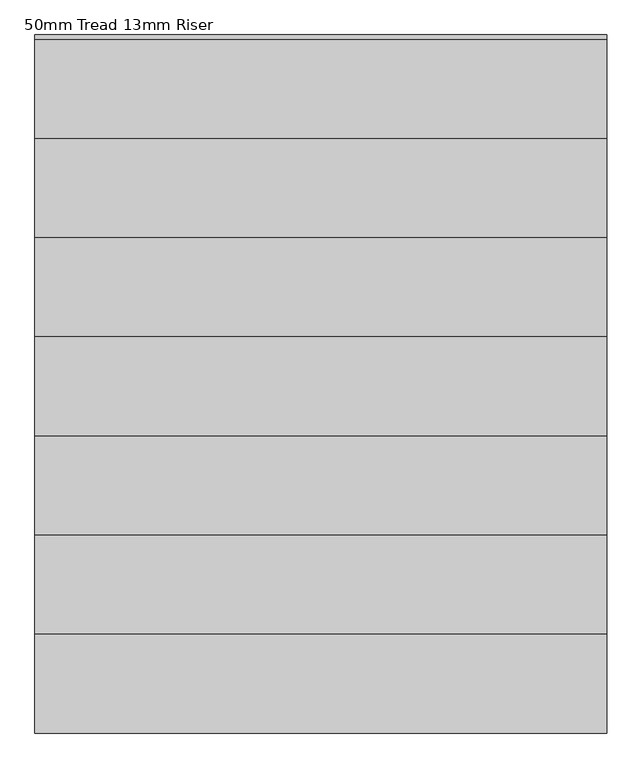
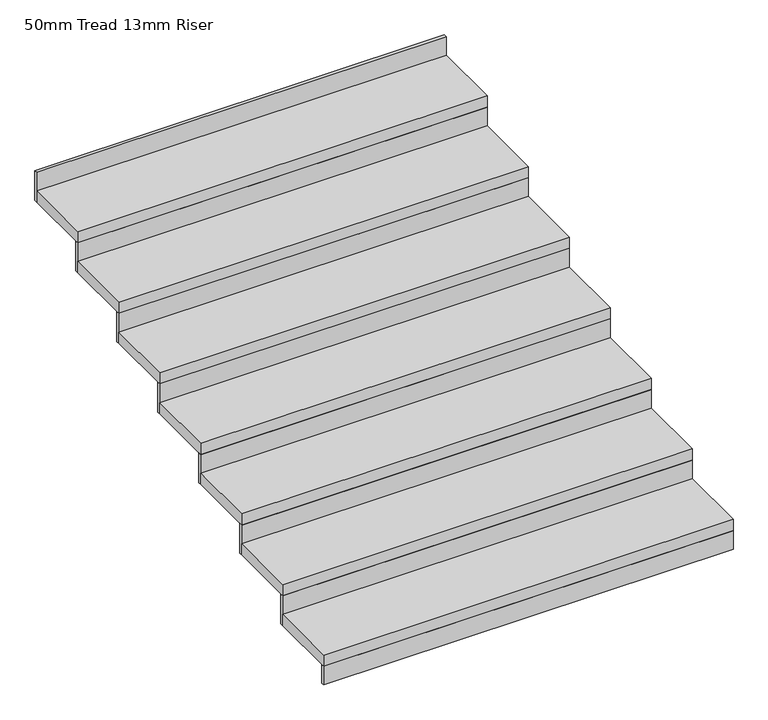
"""IFC4 building model written with IfcOpenShell, lengths in millimetres: stair flight geometry, 50mm Tread 13mm Riser."""

import ifcopenshell
import ifcopenshell.guid

model = None  # the IFC model being written
_history = None  # IfcOwnerHistory: only IFC2X3 demands one
_inside = {}  # id of a spatial element -> (the spatial element, [elements in it])
_under = {}  # id of a project, library or spatial element -> (it, [spatial elements below it])
_declared = {}  # id of a project -> (the project, [libraries it declares])
_typed = {}  # id of a type object -> (the type object, [elements of that type])
_made_of = {}  # id of a material, layer set ... -> (it, [elements and type objects made of it])


def new_model(schema):
    """Start an empty IFC model of exactly this schema.

    Asked for "IFC4X3", IfcOpenShell would pick the latest addendum, in which some entities
    have other attributes; the version numbers below select the first issue.
    IFC2X3 requires an IfcOwnerHistory on every rooted entity: one is made here for all.
    """
    global model, _history
    if schema == "IFC4X3":
        model = ifcopenshell.file(schema_version=(4, 3, 0, 0))
    else:
        model = ifcopenshell.file(schema=schema)
    _inside.clear()
    _under.clear()
    _declared.clear()
    _typed.clear()
    _made_of.clear()
    _history = None
    if model.schema == "IFC2X3":
        org = make("IfcOrganization", Name="unknown")
        user = make(
            "IfcPersonAndOrganization",
            ThePerson=make("IfcPerson", FamilyName="unknown"),
            TheOrganization=org,
        )
        app = make(
            "IfcApplication",
            ApplicationDeveloper=org,
            Version="unknown",
            ApplicationFullName="unknown",
            ApplicationIdentifier="unknown",
        )
        _history = make(
            "IfcOwnerHistory",
            OwningUser=user,
            OwningApplication=app,
            ChangeAction="ADDED",
            CreationDate=0,
        )
    return model


def make(cls, **values):
    """One entity of the class cls with the attributes given. An attribute that is None is left unset."""
    return model.create_entity(
        cls, **{name: value for name, value in values.items() if value is not None}
    )


def rooted(cls, **values):
    """An entity with a GlobalId (a new one), such as an element, a storey or a relation."""
    return make(cls, GlobalId=ifcopenshell.guid.new(), OwnerHistory=_history, **values)


def si_unit(unit_type, name, prefix=None):
    """IfcSIUnit, for example si_unit("LENGTHUNIT", "METRE", prefix="MILLI")."""
    return make("IfcSIUnit", UnitType=unit_type, Prefix=prefix, Name=name)


def assignment(units):
    """IfcUnitAssignment: the units of a project."""
    return None if units is None else make("IfcUnitAssignment", Units=units)


def point(xyz):
    """IfcCartesianPoint."""
    return None if xyz is None else make("IfcCartesianPoint", Coordinates=xyz)


def direction(xyz):
    """IfcDirection."""
    return None if xyz is None else make("IfcDirection", DirectionRatios=xyz)


def frame(location, z_axis=None, x_axis=None):
    """IfcAxis2Placement3D, a coordinate frame: its origin and axes. An axis left out is left unset."""
    return make(
        "IfcAxis2Placement3D",
        Location=point(location),
        Axis=direction(z_axis),
        RefDirection=direction(x_axis),
    )


def origin():
    """The frame at (0, 0, 0) with its axes left unset."""
    return frame((0.0, 0.0, 0.0))


def place(relative_to, where):
    """IfcLocalPlacement: puts the frame where relative to a parent placement (None: the world)."""
    return make(
        "IfcLocalPlacement", PlacementRelTo=relative_to, RelativePlacement=where
    )


def context(
    kind, dimensions, precision=None, world=None, true_north=None, identifier=None
):
    """IfcGeometricRepresentationContext, for example the 3D "Model" context."""
    return make(
        "IfcGeometricRepresentationContext",
        ContextIdentifier=identifier,
        ContextType=kind,
        CoordinateSpaceDimension=dimensions,
        Precision=precision,
        WorldCoordinateSystem=world,
        TrueNorth=true_north,
    )


def project(units=None, contexts=None):
    """IfcProject with its units and contexts."""
    return rooted(
        "IfcProject",
        Name="project",
        RepresentationContexts=contexts,
        UnitsInContext=assignment(units),
    )


def spatial(cls, under=None, at=None, **own):
    """A site, building, storey or space (cls), placed at a placement, below another one or the project."""
    s = rooted(cls, ObjectPlacement=at, **own)
    if under is not None:
        _under.setdefault(under.id(), (under, []))[1].append(s)
    return s


def polyline(points):
    """IfcPolyline through the points."""
    return make("IfcPolyline", Points=[point(p) for p in points])


def outline(outer, holes=None, kind="AREA"):
    """IfcArbitraryClosedProfileDef: a profile drawn as a closed curve; with holes, ...WithVoids."""
    if holes is None:
        return make("IfcArbitraryClosedProfileDef", ProfileType=kind, OuterCurve=outer)
    return make(
        "IfcArbitraryProfileDefWithVoids",
        ProfileType=kind,
        OuterCurve=outer,
        InnerCurves=holes,
    )


def extrude(swept, where, along, depth):
    """IfcExtrudedAreaSolid: the profile swept, set in the frame where, extruded along a direction by depth."""
    return make(
        "IfcExtrudedAreaSolid",
        SweptArea=swept,
        Position=where,
        ExtrudedDirection=direction(along),
        Depth=depth,
    )


def shape(context_of_items, identifier, shape_type, items):
    """IfcShapeRepresentation: the items that make up one representation, for example the "Body"."""
    return make(
        "IfcShapeRepresentation",
        ContextOfItems=context_of_items,
        RepresentationIdentifier=identifier,
        RepresentationType=shape_type,
        Items=items,
    )


def source(mapping_origin, context_of_items, identifier, shape_type, items):
    """IfcRepresentationMap: a shape defined once, which mapped items show again and again."""
    return make(
        "IfcRepresentationMap",
        MappingOrigin=mapping_origin,
        MappedRepresentation=shape(context_of_items, identifier, shape_type, items),
    )


def transform(
    local_origin,
    x_axis=None,
    y_axis=None,
    z_axis=None,
    scale=None,
    scale2=None,
    scale3=None,
    uniform=True,
):
    """IfcCartesianTransformationOperator3D, or its non-uniform kind. x_axis, y_axis, z_axis: its Axis1, 2, 3."""
    if uniform:
        return make(
            "IfcCartesianTransformationOperator3D",
            Axis1=direction(x_axis),
            Axis2=direction(y_axis),
            LocalOrigin=point(local_origin),
            Scale=scale,
            Axis3=direction(z_axis),
        )
    return make(
        "IfcCartesianTransformationOperator3DnonUniform",
        Axis1=direction(x_axis),
        Axis2=direction(y_axis),
        LocalOrigin=point(local_origin),
        Scale=scale,
        Axis3=direction(z_axis),
        Scale2=scale2,
        Scale3=scale3,
    )


def mapped(mapping_source, mapping_target):
    """IfcMappedItem: shows the shape of a source again, moved by a transform."""
    return make(
        "IfcMappedItem", MappingSource=mapping_source, MappingTarget=mapping_target
    )


def made_of(thing, what):
    """Note that an element or type object is made of a material, layer set ...; save() writes the relation."""
    if what is not None:
        _made_of.setdefault(what.id(), (what, []))[1].append(thing)
    return thing


def element(
    cls,
    number,
    at=None,
    inside=None,
    cuts=None,
    type_object=None,
    material=None,
    context=None,
    identifier="Body",
    shape_type=None,
    held_by="IfcProductDefinitionShape",
    body=None,
    shapes=None,
    **own,
):
    """One element of the class cls, such as IfcWall. Its Tag is "e" and its number.

    at: its placement. inside: the storey or other place that contains it. cuts: it is an
    opening in that element (IfcRelVoidsElement). A single representation is given by context,
    identifier, shape_type and body (its items); several are given by shapes. held_by: the class
    of the entity that holds the representations. save() writes the other relations.
    """
    e = rooted(cls, Tag="e%d" % number, ObjectPlacement=at, **own)
    if body is not None:
        shapes = [shape(context, identifier, shape_type, body)]
    if shapes is not None:
        e.Representation = make(held_by, Representations=shapes)
    if inside is not None:
        _inside.setdefault(inside.id(), (inside, []))[1].append(e)
    if cuts is not None:
        rooted(
            "IfcRelVoidsElement", RelatingBuildingElement=cuts, RelatedOpeningElement=e
        )
    if type_object is not None:
        _typed.setdefault(type_object.id(), (type_object, []))[1].append(e)
    return made_of(e, material)


def aggregate(whole, parts):
    """IfcRelAggregates: a whole, such as a stair, and the parts it consists of."""
    return rooted("IfcRelAggregates", RelatingObject=whole, RelatedObjects=parts)


def save(model, path):
    """Write the relations noted so far, then the file.

    IfcRelAggregates (storeys below a building ...), IfcRelContainedInSpatialStructure (elements
    in a storey), IfcRelDefinesByType, IfcRelAssociatesMaterial and IfcRelDeclares: one each for
    every whole, place, type object, material and project.
    """
    for whole, parts in _under.values():
        aggregate(whole, parts)
    for where, things in _inside.values():
        rooted(
            "IfcRelContainedInSpatialStructure",
            RelatedElements=things,
            RelatingStructure=where,
        )
    for kind, things in _typed.values():
        rooted("IfcRelDefinesByType", RelatedObjects=things, RelatingType=kind)
    for what, things in _made_of.values():
        rooted("IfcRelAssociatesMaterial", RelatedObjects=things, RelatingMaterial=what)
    for by, libraries in _declared.values():
        rooted("IfcRelDeclares", RelatingContext=by, RelatedDefinitions=libraries)
    model.write(path)


def stair_flight_50mm_tread_13mm_riser_0aac887c(model_context):
    return source(origin(), model_context, "Body", "SweptSolid", [
        extrude(outline(polyline([(-15644.418089, 13093.1768963), (-15644.418089, 13080.6768963), (-17374.418089, 13080.6768963), (-17374.418089, 13093.1768963), (-15644.418089, 13093.1768963)])), frame((0.0, 0.0, -2133.3333333), z_axis=(0.0, 0.0, 1.0), x_axis=(1.0, 0.0, 0.0)), (0.0, 0.0, 1.0), 83.3333333),
        extrude(outline(polyline([(-17374.418089, 13380.6768963), (-15644.418089, 13380.6768963), (-15644.418089, 13080.6768963), (-17374.418089, 13080.6768963), (-17374.418089, 13380.6768963)])), frame((0.0, 0.0, -2050.0), z_axis=(0.0, 0.0, 1.0), x_axis=(1.0, 0.0, 0.0)), (0.0, 0.0, 1.0), 50.0),
        extrude(outline(polyline([(-15644.418089, 13393.1768963), (-15644.418089, 13380.6768963), (-17374.418089, 13380.6768963), (-17374.418089, 13393.1768963), (-15644.418089, 13393.1768963)])), frame((0.0, 0.0, -2050.0), z_axis=(0.0, 0.0, 1.0), x_axis=(1.0, 0.0, 0.0)), (0.0, 0.0, 1.0), 133.3333333),
        extrude(outline(polyline([(-17374.418089, 13680.6768963), (-15644.418089, 13680.6768963), (-15644.418089, 13380.6768963), (-17374.418089, 13380.6768963), (-17374.418089, 13680.6768963)])), frame((0.0, 0.0, -1916.6666667), z_axis=(0.0, 0.0, 1.0), x_axis=(1.0, 0.0, 0.0)), (0.0, 0.0, 1.0), 50.0),
        extrude(outline(polyline([(-15644.418089, 13693.1768963), (-15644.418089, 13680.6768963), (-17374.418089, 13680.6768963), (-17374.418089, 13693.1768963), (-15644.418089, 13693.1768963)])), frame((0.0, 0.0, -1916.6666667), z_axis=(0.0, 0.0, 1.0), x_axis=(1.0, 0.0, 0.0)), (0.0, 0.0, 1.0), 133.3333333),
        extrude(outline(polyline([(-17374.418089, 13980.6768963), (-15644.418089, 13980.6768963), (-15644.418089, 13680.6768963), (-17374.418089, 13680.6768963), (-17374.418089, 13980.6768963)])), frame((0.0, 0.0, -1783.3333333), z_axis=(0.0, 0.0, 1.0), x_axis=(1.0, 0.0, 0.0)), (0.0, 0.0, 1.0), 50.0),
        extrude(outline(polyline([(-15644.418089, 13993.1768963), (-15644.418089, 13980.6768963), (-17374.418089, 13980.6768963), (-17374.418089, 13993.1768963), (-15644.418089, 13993.1768963)])), frame((0.0, 0.0, -1783.3333333), z_axis=(0.0, 0.0, 1.0), x_axis=(1.0, 0.0, 0.0)), (0.0, 0.0, 1.0), 133.3333333),
        extrude(outline(polyline([(-17374.418089, 14280.6768963), (-15644.418089, 14280.6768963), (-15644.418089, 13980.6768963), (-17374.418089, 13980.6768963), (-17374.418089, 14280.6768963)])), frame((0.0, 0.0, -1650.0), z_axis=(0.0, 0.0, 1.0), x_axis=(1.0, 0.0, 0.0)), (0.0, 0.0, 1.0), 50.0),
        extrude(outline(polyline([(-15644.418089, 14293.1768963), (-15644.418089, 14280.6768963), (-17374.418089, 14280.6768963), (-17374.418089, 14293.1768963), (-15644.418089, 14293.1768963)])), frame((0.0, 0.0, -1650.0), z_axis=(0.0, 0.0, 1.0), x_axis=(1.0, 0.0, 0.0)), (0.0, 0.0, 1.0), 133.3333333),
        extrude(outline(polyline([(-17374.418089, 14580.6768963), (-15644.418089, 14580.6768963), (-15644.418089, 14280.6768963), (-17374.418089, 14280.6768963), (-17374.418089, 14580.6768963)])), frame((0.0, 0.0, -1516.6666667), z_axis=(0.0, 0.0, 1.0), x_axis=(1.0, 0.0, 0.0)), (0.0, 0.0, 1.0), 50.0),
        extrude(outline(polyline([(-15644.418089, 14593.1768963), (-15644.418089, 14580.6768963), (-17374.418089, 14580.6768963), (-17374.418089, 14593.1768963), (-15644.418089, 14593.1768963)])), frame((0.0, 0.0, -1516.6666667), z_axis=(0.0, 0.0, 1.0), x_axis=(1.0, 0.0, 0.0)), (0.0, 0.0, 1.0), 133.3333333),
        extrude(outline(polyline([(-17374.418089, 14880.6768963), (-15644.418089, 14880.6768963), (-15644.418089, 14580.6768963), (-17374.418089, 14580.6768963), (-17374.418089, 14880.6768963)])), frame((0.0, 0.0, -1383.3333333), z_axis=(0.0, 0.0, 1.0), x_axis=(1.0, 0.0, 0.0)), (0.0, 0.0, 1.0), 50.0),
        extrude(outline(polyline([(-15644.418089, 14893.1768963), (-15644.418089, 14880.6768963), (-17374.418089, 14880.6768963), (-17374.418089, 14893.1768963), (-15644.418089, 14893.1768963)])), frame((0.0, 0.0, -1383.3333333), z_axis=(0.0, 0.0, 1.0), x_axis=(1.0, 0.0, 0.0)), (0.0, 0.0, 1.0), 133.3333333),
        extrude(outline(polyline([(-15644.418089, 15193.1768963), (-15644.418089, 15180.6768963), (-17374.418089, 15180.6768963), (-17374.418089, 15193.1768963), (-15644.418089, 15193.1768963)])), frame((0.0, 0.0, -1250.0), z_axis=(0.0, 0.0, 1.0), x_axis=(1.0, 0.0, 0.0)), (0.0, 0.0, 1.0), 133.3333333),
        extrude(outline(polyline([(-17374.418089, 15180.6768963), (-15644.418089, 15180.6768963), (-15644.418089, 14880.6768963), (-17374.418089, 14880.6768963), (-17374.418089, 15180.6768963)])), frame((0.0, 0.0, -1250.0), z_axis=(0.0, 0.0, 1.0), x_axis=(1.0, 0.0, 0.0)), (0.0, 0.0, 1.0), 50.0),
    ])


if __name__ == "__main__":
    model = new_model("IFC4")
    model_context = context("Model", 3, world=origin())
    ifc_project = project(units=[si_unit("LENGTHUNIT", "METRE", prefix="MILLI")], contexts=[model_context])
    site = spatial("IfcSite", under=ifc_project)
    building = spatial("IfcBuilding", under=site)
    placement = place(None, origin())
    stair_flight_50mm_tread_13mm_riser_shape = stair_flight_50mm_tread_13mm_riser_0aac887c(model_context)
    element("IfcStairFlight", 1, ObjectType="50mm Tread 13mm Riser", at=placement, inside=building, context=model_context, shape_type="MappedRepresentation", body=[
        mapped(stair_flight_50mm_tread_13mm_riser_shape, transform((0.0, 0.0, 0.0), x_axis=(1.0, 0.0, 0.0), y_axis=(0.0, 1.0, 0.0), z_axis=(0.0, 0.0, 1.0))),
    ])
    save(model, "model.ifc")
